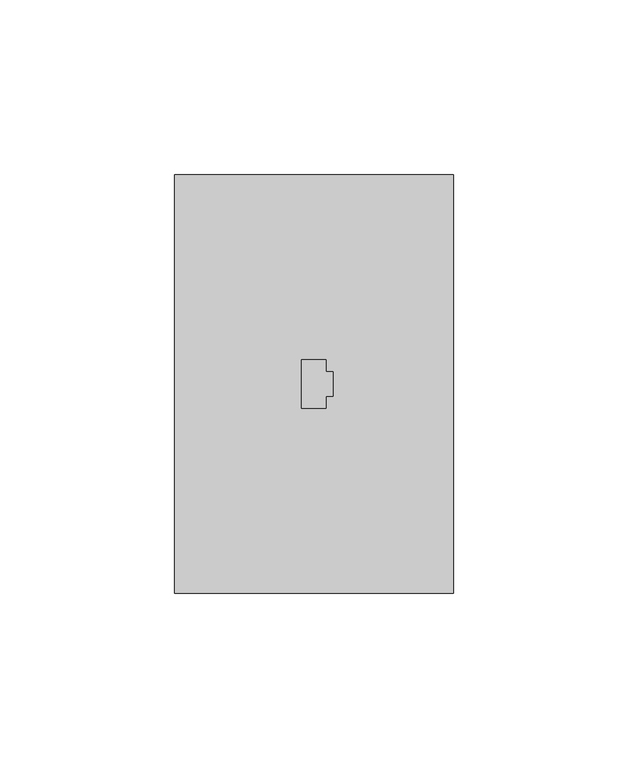
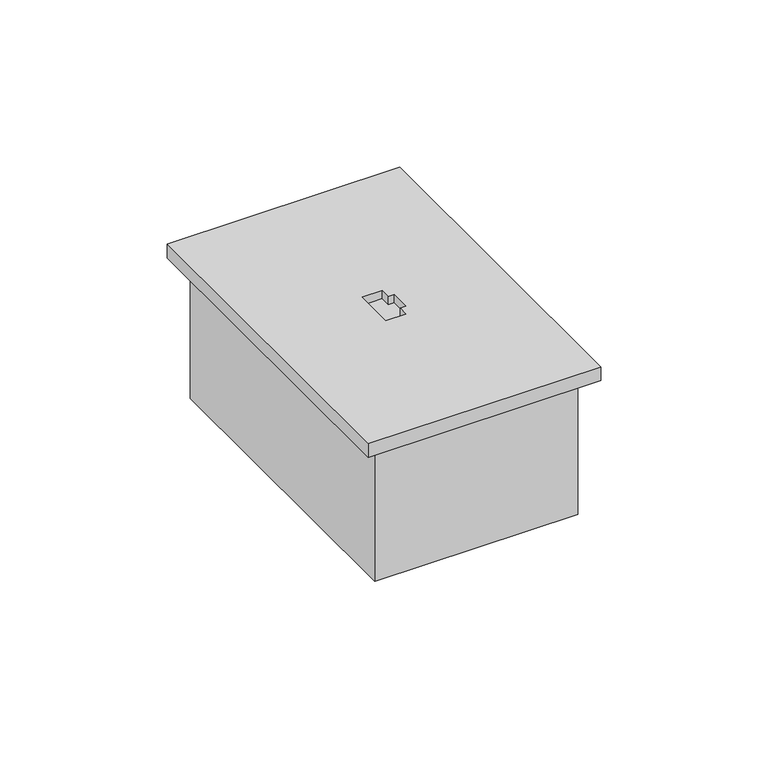
"""IFC4 building model written with IfcOpenShell, lengths in millimetres: proxy geometry, CAIXA VERTICE V7 : Rede."""

from ifc_helpers import new_model, si_unit, origin, place, context, project, spatial, faceted_brep, source, transform, mapped, element, save


def electrical_fixtures_9785a3ee(model_context):
    return source(origin(), model_context, "Body", "Brep", [
        faceted_brep([(33.0, 1047.0, -48.0), (33.0, 1153.0, -48.0), (-33.0, 1153.0, -48.0), (-33.0, 1047.0, -48.0), (35.0, 1155.0, -50.0), (35.0, 1045.0, -50.0), (-35.0, 1045.0, -50.0), (-35.0, 1155.0, -50.0), (-35.0, 1155.0, 0.0), (35.0, 1155.0, 0.0), (-35.0, 1045.0, 0.0), (35.0, 1045.0, 0.0), (33.0, 1153.0, 0.0), (33.0, 1047.0, 0.0), (-33.0, 1047.0, 0.0), (-33.0, 1153.0, 0.0)], [[[0, 1, 2, 3]], [[4, 5, 6, 7]], [[4, 7, 8, 9]], [[8, 7, 6, 10]], [[10, 6, 5, 11]], [[11, 5, 4, 9]], [[9, 8, 10, 11], [12, 13, 14, 15]], [[13, 12, 1, 0]], [[14, 13, 0, 3]], [[15, 14, 3, 2]], [[12, 15, 2, 1]]]),
        faceted_brep([(40.0, 1160.0, 5.0), (-40.0, 1160.0, 5.0), (-40.0, 1040.0, 5.0), (40.0, 1040.0, 5.0), (5.5, 1103.5, 5.0), (5.5, 1096.5, 5.0), (3.5, 1096.5, 5.0), (3.5, 1093.0, 5.0), (-3.5, 1093.0, 5.0), (-3.5, 1107.0, 5.0), (3.5, 1107.0, 5.0), (3.5, 1103.5, 5.0), (-40.0, 1160.0, 0.0), (40.0, 1160.0, 0.0), (40.0, 1040.0, 0.0), (-40.0, 1040.0, 0.0), (5.5, 1103.5, 2.0), (5.5, 1096.5, 2.0), (3.5, 1103.5, 2.0), (3.5, 1107.0, 2.0), (-3.5, 1107.0, 2.0), (-3.5, 1093.0, 2.0), (3.5, 1093.0, 2.0), (3.5, 1096.5, 2.0)], [[[0, 1, 2, 3], [4, 5, 6, 7, 8, 9, 10, 11]], [[12, 13, 14, 15]], [[1, 0, 13, 12]], [[2, 1, 12, 15]], [[3, 2, 15, 14]], [[0, 3, 14, 13]], [[16, 17, 5, 4]], [[18, 16, 4, 11]], [[19, 18, 11, 10]], [[19, 20, 21, 22, 23, 17, 16, 18]], [[20, 19, 10, 9]], [[21, 20, 9, 8]], [[22, 21, 8, 7]], [[23, 22, 7, 6]], [[17, 23, 6, 5]]]),
    ])


if __name__ == "__main__":
    model = new_model("IFC4")
    model_context = context("Model", 3, world=origin())
    ifc_project = project(units=[si_unit("LENGTHUNIT", "METRE", prefix="MILLI")], contexts=[model_context])
    site = spatial("IfcSite", under=ifc_project)
    building = spatial("IfcBuilding", under=site)
    placement = place(None, origin())
    electrical_fixtures_shape = electrical_fixtures_9785a3ee(model_context)
    element("IfcBuildingElementProxy", 1, Name="CAIXA VERTICE V7 : Rede", ObjectType="CAIXA VERTICE V7 : Rede", at=placement, inside=building, context=model_context, shape_type="MappedRepresentation", body=[
        mapped(electrical_fixtures_shape, transform((0.0, 0.0, 0.0), x_axis=(1.0, 0.0, 0.0), y_axis=(0.0, 1.0, 0.0), z_axis=(0.0, 0.0, 1.0))),
    ])
    save(model, "model.ifc")

# Revit data of these elements
# Type "CAIXA VERTICE V7 : Rede"
#   URL = "www.facebook.com/verticetreinamentos"
#   SEÇÃO [instance default] = ""
#   Rotação [instance default] = 0.00°
#   LARGURA DA TAMPA = 0.08 m
#   BORDA = 0.01 m
#   ALTURA DE INSTALAÇÃO [instance default] = 1.10 m
#   Distância Anotação [instance default] = 0.0015 m
#   ALTURA DA TAMPA = 0.12 m
#   Vertical [instance default] = yes
#   VER SEÇÃO [instance default] = no
#   SHADE ESQ [instance default] = no
#   SHADE DIR [instance default] = yes
#   HORIZONTAL [instance default] = no
#   ANDAR COM A LEGENDA [instance default] = 0
#   Material Tampa [instance default] = Plástico, branco opaco
#   Caixa = element 1798521
#   Anotação = element 1798536
#   Default Elevation = 0
# Element 1 (IfcBuildingElementProxy, "CAIXA VERTICE V7 : Rede")
#   Materials on its faces: "Plástico, branco opaco"
# Materials
#   "Plástico, branco opaco": class "Plástico", colour RGB 120 120 120, transparency 0, Description = "Plastic, generic, opaque white", Cost = 0
